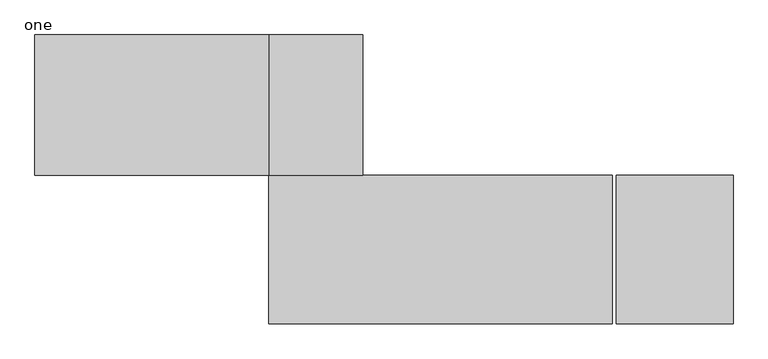
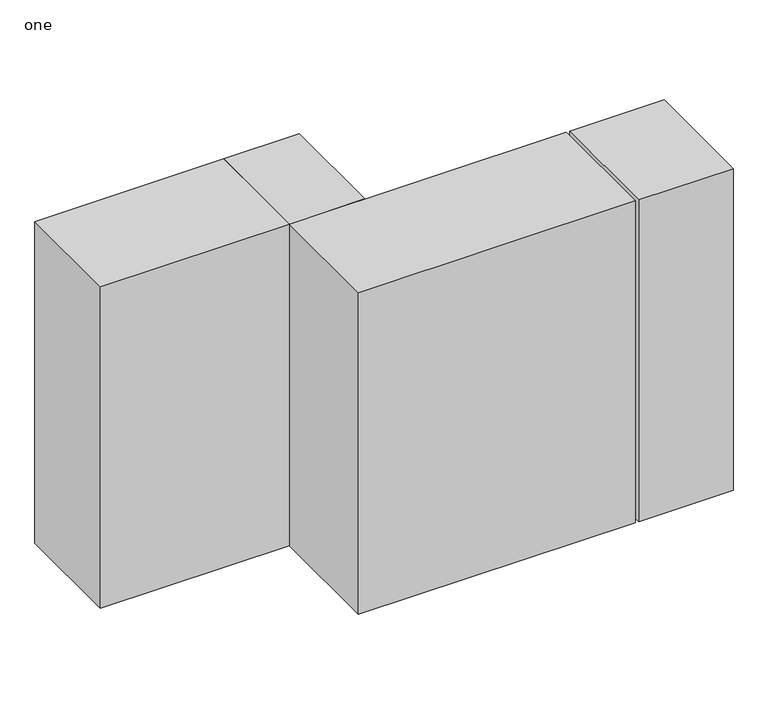
"""IFC4 building model written with IfcOpenShell, lengths in millimetres: proxy geometry, Canner : one."""

from ifc_helpers import new_model, si_unit, origin, origin_with_axes, place, context, project, spatial, polyline, outline, extrude, source, transform, mapped, element, save


def one_8a4aaae7(model_context):
    return source(origin(), model_context, "Body", "SweptSolid", [
        extrude(outline(polyline([(-1117.6, 482.6), (-2641.6, 482.6), (-2641.6, 1397.0), (-1117.6, 1397.0), (-1117.6, 482.6)])), origin_with_axes(), (0.0, 0.0, 1.0), 2743.2),
        extrude(outline(polyline([(-508.0, 482.6), (-1117.6, 482.6), (-1117.6, 1397.0), (-508.0, 1397.0), (-508.0, 482.6)])), origin_with_axes(), (0.0, 0.0, 1.0), 2743.2),
        extrude(outline(polyline([(1905.0, -482.6), (1143.0, -482.6), (1143.0, 482.6), (1905.0, 482.6), (1905.0, -482.6)])), origin_with_axes(), (0.0, 0.0, 1.0), 2743.2),
        extrude(outline(polyline([(1117.6, -482.6), (-1117.6, -482.6), (-1117.6, 482.6), (1117.6, 482.6), (1117.6, -482.6)])), origin_with_axes(), (0.0, 0.0, 1.0), 2743.2),
    ])


if __name__ == "__main__":
    model = new_model("IFC4")
    model_context = context("Model", 3, world=origin())
    ifc_project = project(units=[si_unit("LENGTHUNIT", "METRE", prefix="MILLI")], contexts=[model_context])
    site = spatial("IfcSite", under=ifc_project)
    building = spatial("IfcBuilding", under=site)
    placement = place(None, origin())
    one_shape = one_8a4aaae7(model_context)
    element("IfcBuildingElementProxy", 1, Name="Canner : one", ObjectType="Canner : one", at=placement, inside=building, context=model_context, shape_type="MappedRepresentation", body=[
        mapped(one_shape, transform((0.0, 0.0, 0.0), x_axis=(1.0, 0.0, 0.0), y_axis=(0.0, 1.0, 0.0), z_axis=(0.0, 0.0, 1.0))),
    ])
    save(model, "model.ifc")

# Revit data of these elements
# Type "Canner : one"
#   Width = 3' - 2"
#   Length = 7' - 4"
#   Height = 9' - 0"
#   Table = CANNING TABLE
#   Outfeed Table = SORTING/PACKING TABLE
#   Feeder = WHALE TAIL FEEDER
#   Dunk Tank = DUNK TANK
# Element 1 (IfcBuildingElementProxy, "Canner : one")
#   Materials on its faces: "SORTING/PACKING TABLE", "DUNK TANK", "WHALE TAIL FEEDER", "CANNING TABLE"
# Materials
#   "CANNING TABLE": class "Generic", colour RGB 181 181 181, transparency 0, Cost = 0
#   "SORTING/PACKING TABLE": class "Generic", colour RGB 181 181 181, transparency 0, Cost = 0
#   "WHALE TAIL FEEDER": class "Generic", colour RGB 181 181 181, transparency 0, Cost = 0
#   "DUNK TANK": class "Generic", colour RGB 181 181 181, transparency 0, Cost = 0
